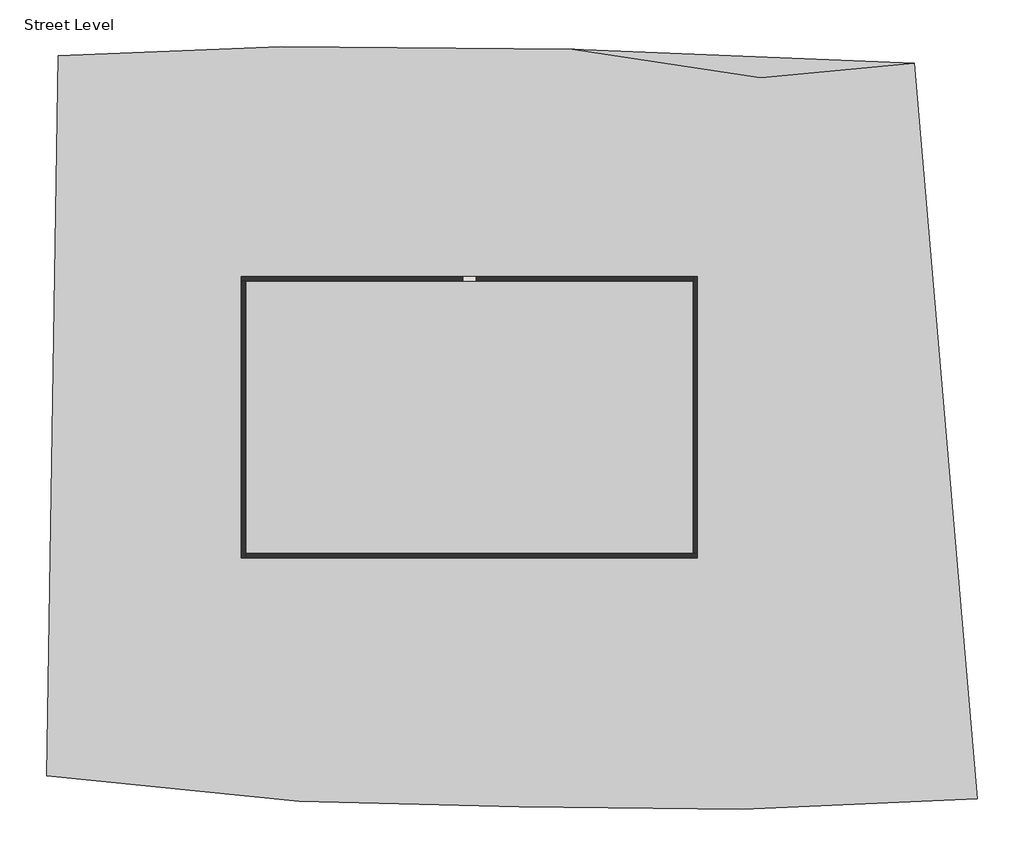
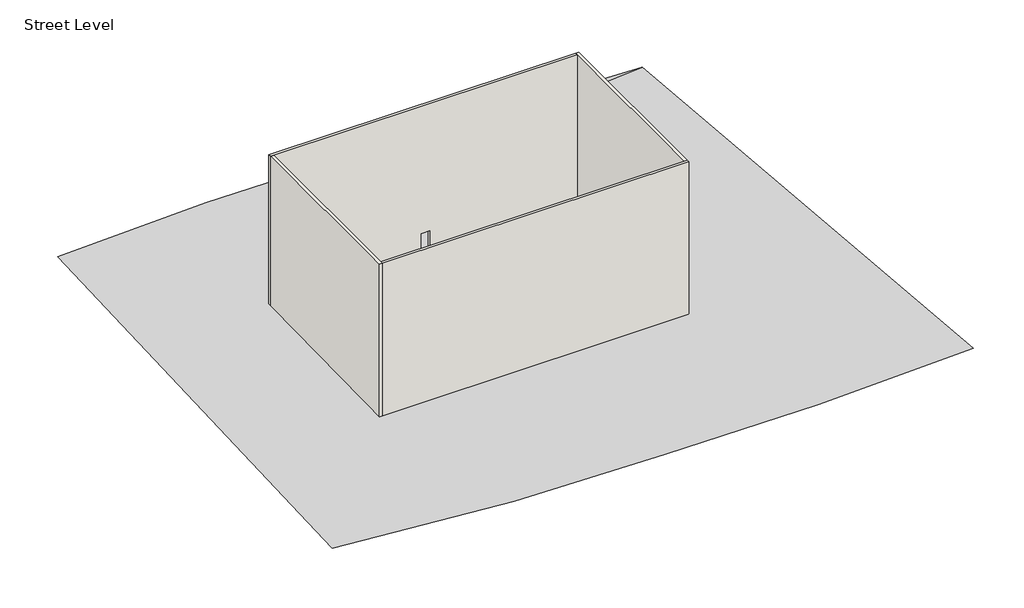
# One storey: 4 walls, 1 proxy.
"""IFC4 building model written with IfcOpenShell, lengths in millimetres."""

from ifc_helpers import new_model, si_unit, origin, place, context, project, spatial, faceted_brep, triangles, element, save

model = new_model("IFC4")

# Units and contexts
model_context = context("Model", 3, world=origin())
ifc_project = project(units=[si_unit("LENGTHUNIT", "METRE", prefix="MILLI")], contexts=[model_context])

# Site, building, storey
site = spatial("IfcSite", under=ifc_project)
building = spatial("IfcBuilding", under=site)
storey = spatial("IfcBuildingStorey", under=building, Name="Street Level", Elevation=-914.4)

# Proxy
placement = place(None, origin())
element("IfcBuildingElementProxy", 1, Name="Building Element Proxy", at=placement, inside=storey, context=model_context, shape_type="Tessellation", body=[
    triangles([(-29664.1428223, 25063.2445862, 0.0), (-14195.9393097, 25689.5644958, 0.0), (5935.7725708, 25510.6149536, 0.0), (18999.0170654, 23542.1816162, 0.0), (29646.4555298, 24526.3982849, 0.0), (-30469.4122742, -24863.4009705, -914.4), (-12943.2994904, -26652.8870911, -914.4), (2267.3273026, -27010.7838501, -914.4), (17746.3772461, -27189.7333923, -914.4), (34030.6948975, -26473.9375488, -914.4)], [[7, 8, 2], [6, 2, 1], [2, 6, 7], [8, 3, 2], [9, 10, 4], [3, 4, 5], [3, 8, 4], [5, 4, 10], [4, 8, 9]], closed=False),
])

# Walls
element("IfcWall", 2, ObjectType="Generic - 12\"", at=placement, inside=storey, context=model_context, shape_type="Brep", body=[
    faceted_brep([(-16964.6122732, 9443.9015304, -914.4), (-16659.8122732, 9443.9015304, -914.4), (14328.1877268, 9443.9015304, -914.4), (14328.1877268, 9443.9015304, 15849.6), (-16659.8122732, 9443.9015304, 15849.6), (-16964.6122732, 9443.9015304, 15849.6), (-708.6122732, 9443.9015304, 0.0), (-1623.0122732, 9443.9015304, 0.0), (-1623.0122732, 9443.9015304, 2133.6), (-708.6122732, 9443.9015304, 2133.6), (-16964.6122732, 9748.7015304, -914.4), (-16964.6122732, 9748.7015304, 15849.6), (14328.1877268, 9748.7015304, 15849.6), (14328.1877268, 9748.7015304, -914.4), (-708.6122732, 9748.7015304, 0.0), (-708.6122732, 9748.7015304, 2133.6), (-1623.0122732, 9748.7015304, 2133.6), (-1623.0122732, 9748.7015304, 0.0)], [[[0, 1, 2, 3, 4, 5], [6, 7, 8, 9]], [[10, 11, 12, 13], [14, 15, 16, 17]], [[2, 1, 0, 10, 13]], [[5, 4, 3, 12, 11]], [[0, 5, 11, 10]], [[3, 2, 13, 12]], [[7, 6, 14, 17]], [[8, 7, 17, 16]], [[9, 8, 16, 15]], [[6, 9, 15, 14]]]),
])
element("IfcWall", 3, ObjectType="Generic - 12\"", at=placement, inside=storey, context=model_context, shape_type="Brep", body=[
    faceted_brep([(-16659.8122732, -9758.4984696, -914.4), (-16659.8122732, -9453.6984696, -914.4), (-16659.8122732, 9443.9015304, -914.4), (-16659.8122732, 9443.9015304, 15849.6), (-16659.8122732, -9453.6984696, 15849.6), (-16659.8122732, -9758.4984696, 15849.6), (-16964.6122732, -9758.4984696, -914.4), (-16964.6122732, -9758.4984696, 15849.6), (-16964.6122732, 9443.9015304, 15849.6), (-16964.6122732, 9443.9015304, -914.4)], [[[0, 1, 2, 3, 4, 5]], [[6, 7, 8, 9]], [[2, 1, 0, 6, 9]], [[5, 4, 3, 8, 7]], [[0, 5, 7, 6]], [[3, 2, 9, 8]]]),
])
element("IfcWall", 4, ObjectType="Generic - 12\"", at=placement, inside=storey, context=model_context, shape_type="Brep", body=[
    faceted_brep([(14632.9877268, -9453.6984696, -914.4), (14328.1877268, -9453.6984696, -914.4), (-16659.8122732, -9453.6984696, -914.4), (-16659.8122732, -9453.6984696, 15849.6), (14328.1877268, -9453.6984696, 15849.6), (14632.9877268, -9453.6984696, 15849.6), (14632.9877268, -9758.4984696, -914.4), (14632.9877268, -9758.4984696, 15849.6), (-16659.8122732, -9758.4984696, 15849.6), (-16659.8122732, -9758.4984696, -914.4)], [[[0, 1, 2, 3, 4, 5]], [[6, 7, 8, 9]], [[2, 1, 0, 6, 9]], [[5, 4, 3, 8, 7]], [[0, 5, 7, 6]], [[3, 2, 9, 8]]]),
])
element("IfcWall", 5, ObjectType="Generic - 12\"", at=placement, inside=storey, context=model_context, shape_type="Brep", body=[
    faceted_brep([(14328.1877268, 9748.7015304, -914.4), (14328.1877268, 9443.9015304, -914.4), (14328.1877268, -9453.6984696, -914.4), (14328.1877268, -9453.6984696, 15849.6), (14328.1877268, 9443.9015304, 15849.6), (14328.1877268, 9748.7015304, 15849.6), (14632.9877268, 9748.7015304, -914.4), (14632.9877268, 9748.7015304, 15849.6), (14632.9877268, -9453.6984696, 15849.6), (14632.9877268, -9453.6984696, -914.4)], [[[0, 1, 2, 3, 4, 5]], [[6, 7, 8, 9]], [[2, 1, 0, 6, 9]], [[5, 4, 3, 8, 7]], [[0, 5, 7, 6]], [[3, 2, 9, 8]]]),
])

save(model, "model.ifc")

# Revit data of these elements
# Project information
#   Organization Name = "G3B Press"
#   Organization Description = "Paul F. Aubin Cosulting Services, Inc."
#   Building Name = "Revit Essentials for Architecture"
#   Author = "Paul F. Aubin"
#   Author Website = "https://www.paulaubin.com"
#   Copyright = "Copyright © 2020 Paul F Aubin, all rights reserved"
#   Project Issue Date = "8/1/2020"
#   Project Status = "Design Development"
#   Client Name = "Column Grids and Structural Layout"
#   Project Address = "123 State ST\nSuite 301\nChicago, IL 60606"
#   Project Name = "06 Commercial"
#   Project Number = "2020.04A"
# Type "Generic - 12\""
#   Assembly Code = "B2010"
#   Layers, outside or top first: 1' - 0" no material (function 1)
# Element 1 (IfcBuildingElementProxy)
#   Material = none
#   Phase Created = New Construction
# Elements 2, 3, 4, 5 (IfcWall, "Generic - 12\"")
#   Top Offset = 4' - 0"
#   Base Offset = 0' - 0"
#   wall height = 55' - 0"
#   Phase Created = New Construction
#   Base Constraint = Street Level
#   Top Constraint = Roof
#   Materials on its faces: "Default Wall"
# Materials
#   "Default Wall": class "Miscellaneous", colour RGB 128 128 128, transparency 0, Cost = 0
